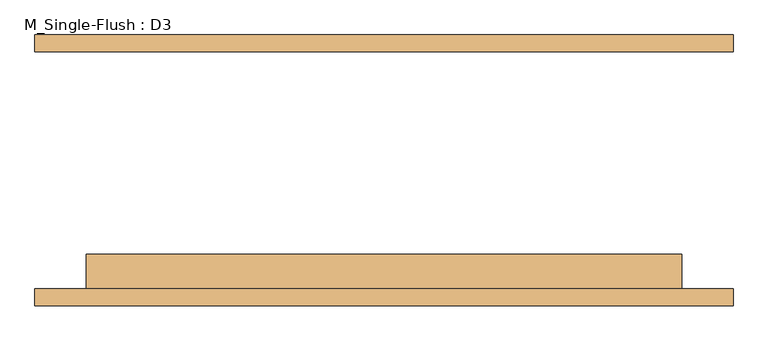
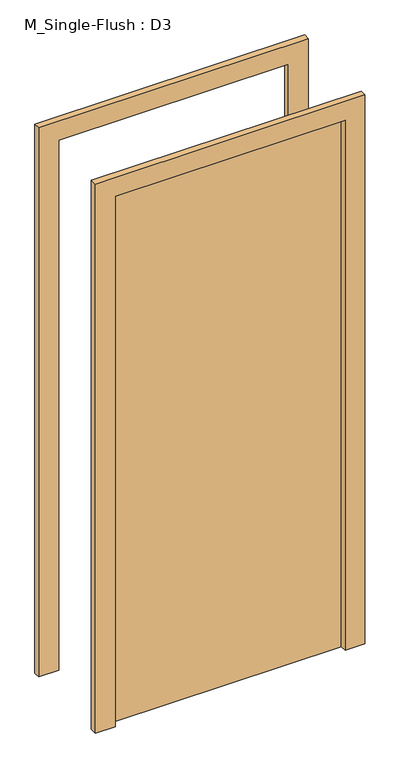
"""IFC4 building model written with IfcOpenShell, lengths in millimetres: door geometry, M_Single-Flush : D3."""

from ifc_helpers import new_model, si_unit, frame, origin, origin_with_axes, place, context, project, spatial, polyline, outline, extrude, source, transform, mapped, element, save


def m_single_flush_d3_71e413c5(model_context):
    return source(origin(), model_context, "Body", "SweptSolid", [
        extrude(outline(polyline([(2221.0, -516.0), (0.0, -516.0), (0.0, -440.0), (2145.0, -440.0), (2145.0, 440.0), (0.0, 440.0), (0.0, 516.0), (2221.0, 516.0), (2221.0, -516.0)])), frame((0.0, -200.0, 0.0), z_axis=(0.0, 1.0, 0.0), x_axis=(0.0, 0.0, 1.0)), (0.0, 0.0, 1.0), 25.0),
        extrude(outline(polyline([(2221.0, 516.0), (2221.0, -516.0), (0.0, -516.0), (0.0, -440.0), (2145.0, -440.0), (2145.0, 440.0), (0.0, 440.0), (0.0, 516.0), (2221.0, 516.0)])), frame((0.0, 175.0, 0.0), z_axis=(0.0, 1.0, 0.0), x_axis=(0.0, 0.0, 1.0)), (0.0, 0.0, 1.0), 25.0),
        extrude(outline(polyline([(440.0, -124.0), (440.0, -175.0), (-440.0, -175.0), (-440.0, -124.0), (440.0, -124.0)])), origin_with_axes(), (0.0, 0.0, 1.0), 2145.0),
    ])


if __name__ == "__main__":
    model = new_model("IFC4")
    model_context = context("Model", 3, world=origin())
    ifc_project = project(units=[si_unit("LENGTHUNIT", "METRE", prefix="MILLI")], contexts=[model_context])
    site = spatial("IfcSite", under=ifc_project)
    building = spatial("IfcBuilding", under=site)
    placement = place(None, origin())
    m_single_flush_d3_shape = m_single_flush_d3_71e413c5(model_context)
    element("IfcDoor", 1, ObjectType="M_Single-Flush : D3", at=placement, inside=building, context=model_context, shape_type="MappedRepresentation", body=[
        mapped(m_single_flush_d3_shape, transform((0.0, 0.0, 0.0), x_axis=(1.0, 0.0, 0.0), y_axis=(0.0, 1.0, 0.0), z_axis=(0.0, 0.0, 1.0))),
    ])
    save(model, "model.ifc")

# Revit data of these elements
# Type "M_Single-Flush : D3"
#   Type Mark = "22"
#   Thickness = 51 mm
#   Height = 2145 mm
#   Trim Projection Ext = 25 mm
#   Trim Projection Int = 25 mm
#   Trim Width = 76 mm
#   Width = 880 mm
#   Door Material = Door - Panel
#   Frame Material = Door - Frame
#   Function = (empty or 0)
#   Wall Closure = (empty or 0)
# Element 1 (IfcDoor, "M_Single-Flush : D3")
#   Materials on its faces: "Door - Frame", "Door - Panel"
# Materials
#   "Door - Panel": class "Wood", colour RGB 210 159 95, transparency 0
#   "Door - Frame": class "Miscellaneous", colour RGB 118 70 51, transparency 0
